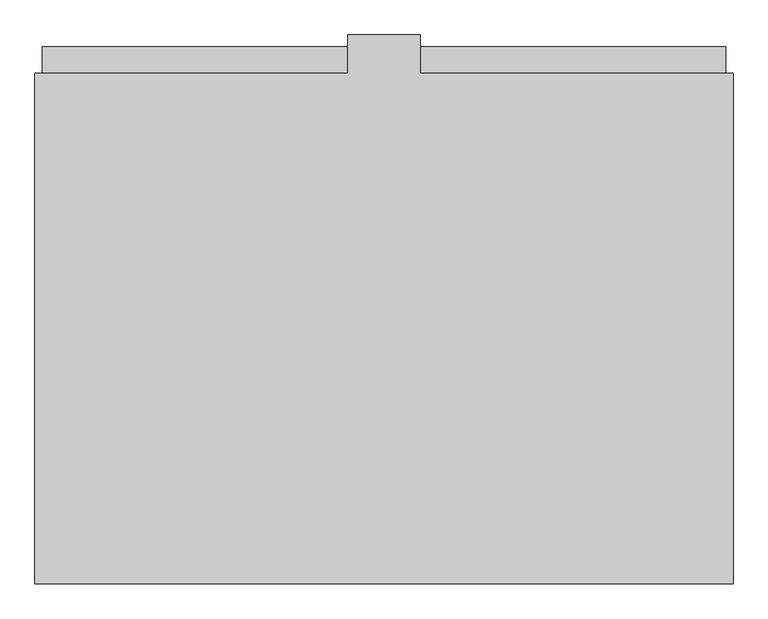
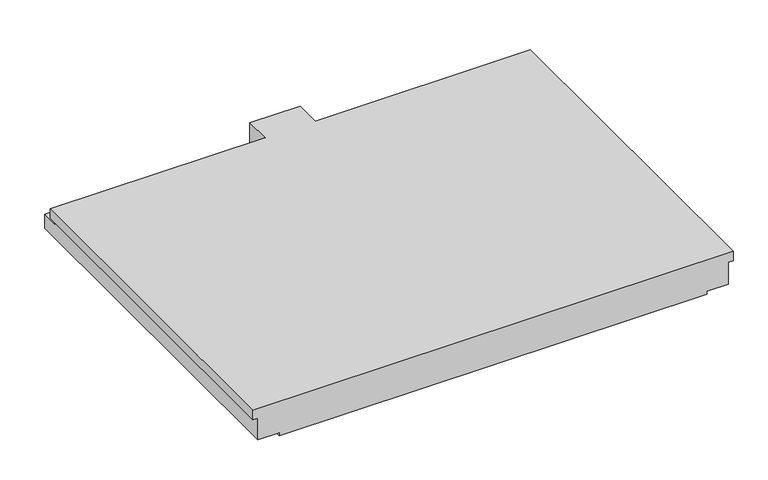
"""IFC4 building model written with IfcOpenShell, lengths in millimetres: proxy geometry, NLRS_24_GM_UN_rechthoekig bordes prefab-AV_gen_rsf : prefab bordes_gen__2250x2925."""

from ifc_helpers import new_model, si_unit, origin, place, context, project, spatial, faceted_brep, source, transform, mapped, element, save


def generic_models_0f5fce95(model_context):
    return source(origin(), model_context, "Body", "Brep", [
        faceted_brep([(1462.5, 2140.0, 0.0), (1462.5, 0.0, 0.0), (1462.5, 0.0, -60.0), (1462.5, 2140.0, -60.0), (152.5, 2250.0, -110.0), (152.5, 2140.0, -110.0), (1432.5, 2140.0, -110.0), (1432.5, 2250.0, -110.0), (152.5, 2140.0, 0.0), (1432.5, 2140.0, -60.0), (152.5, 2300.0, -220.0), (152.5, 2300.0, 0.0), (152.5, 2250.0, -220.0), (-152.5, 2300.0, 0.0), (-152.5, 2300.0, -220.0), (-152.5, 2250.0, -220.0), (-152.5, 2250.0, -110.0), (-152.5, 2140.0, -110.0), (-152.5, 2140.0, 0.0), (-1462.5, 0.0, 0.0), (-1462.5, 2140.0, 0.0), (-1462.5, 2140.0, -60.0), (-1462.5, 0.0, -60.0), (-1302.5, 2250.0, -220.0), (-1302.5, 2250.0, -200.0), (-1432.5, 2250.0, -200.0), (-1432.5, 2250.0, -110.0), (-1432.5, 2140.0, -110.0), (-1432.5, 2140.0, -60.0), (-1432.5, 0.0, -60.0), (-1432.5, 0.0, -200.0), (-1302.5, 0.0, -200.0), (-1302.5, 0.0, -220.0), (1302.5, 0.0, -220.0), (1302.5, 0.0, -200.0), (1432.5, 0.0, -200.0), (1432.5, 0.0, -60.0), (1302.5, 2250.0, -220.0), (1432.5, 2250.0, -200.0), (1302.5, 2250.0, -200.0)], [[[0, 1, 2, 3]], [[4, 5, 6, 7]], [[8, 0, 3, 9, 6, 5]], [[10, 11, 8, 5, 4, 12]], [[13, 14, 15, 16, 17, 18]], [[19, 20, 21, 22]], [[15, 23, 24, 25, 26, 16]], [[16, 26, 27, 17]], [[20, 18, 17, 27, 28, 21]], [[20, 19, 1, 0, 8, 11, 13, 18]], [[19, 22, 29, 30, 31, 32, 33, 34, 35, 36, 2, 1]], [[23, 15, 14, 10, 12, 37, 33, 32]], [[28, 29, 22, 21]], [[25, 30, 29, 28, 27, 26]], [[30, 25, 24, 31]], [[31, 24, 23, 32]], [[36, 9, 3, 2]], [[9, 36, 35, 38, 7, 6]], [[38, 35, 34, 39]], [[39, 34, 33, 37]], [[12, 4, 7, 38, 39, 37]], [[11, 10, 14, 13]]]),
    ])


if __name__ == "__main__":
    model = new_model("IFC4")
    model_context = context("Model", 3, world=origin())
    ifc_project = project(units=[si_unit("LENGTHUNIT", "METRE", prefix="MILLI")], contexts=[model_context])
    site = spatial("IfcSite", under=ifc_project)
    building = spatial("IfcBuilding", under=site)
    placement = place(None, origin())
    generic_models_shape = generic_models_0f5fce95(model_context)
    element("IfcBuildingElementProxy", 1, Name="NLRS_24_GM_UN_rechthoekig bordes prefab-AV_gen_rsf : prefab bordes_gen__2250x2925", ObjectType="NLRS_24_GM_UN_rechthoekig bordes prefab-AV_gen_rsf : prefab bordes_gen__2250x2925", at=placement, inside=building, context=model_context, shape_type="MappedRepresentation", body=[
        mapped(generic_models_shape, transform((0.0, 0.0, 0.0), x_axis=(1.0, 0.0, 0.0), y_axis=(0.0, 1.0, 0.0), z_axis=(0.0, 0.0, 1.0))),
    ])
    save(model, "model.ifc")

# Revit data of these elements
# Type "NLRS_24_GM_UN_rechthoekig bordes prefab-AV_gen_rsf : prefab bordes_gen__2250x2925"
#   Export Type to IFC As = "IfcStair"
#   Type IfcGUID = "2CEqVLPNH8KRN7ghwV3bMM"
#   Type Comments = " "
#   Model = " "
#   Manufacturer = " "
#   Description = "rechthoekig bordes prefab\r\n1930x4395"
#   Assembly Code = "24.15"
#   Width = 2925 mm
#   Thickness = 220 mm
#   Perimeter = 10450 mm
#   NLRS_C_lengte_02 = 1310 mm
#   NLRS_C_lengte_01 = 1310 mm
#   NLRS_C_hoogte_02 = 110 mm
#   NLRS_C_hoogte_01 = 110 mm
#   NLRS_C_diepte_04 = 2250 mm
#   NLRS_C_diepte_03 = 2250 mm
#   NLRS_C_diepte_02 = 110 mm
#   NLRS_C_diepte_01 = 110 mm
#   Length = 2300 mm
#   Default Elevation = 1219.2 mm
#   Area = 6.7275 m²
#   NLRS_C_materiaal = NLRS_f2_beton prefab_gen_rsf
#   Keynote = ""
# Element 1 (IfcBuildingElementProxy, "NLRS_24_GM_UN_rechthoekig bordes prefab-AV_gen_rsf : prefab bordes_gen__2250x2925")
#   Materials on its faces: "NLRS_f2_beton prefab_gen_rsf"
# Materials
#   "NLRS_f2_beton prefab_gen_rsf": class "F - Niet gebakken kunststeen", colour RGB 129 133 118, transparency 0, Keynote = "f2", Manufacturer = "Revit Standards Foundation", URL = "www.revitstandards.org", Description = "beton prefab", Cost = 0
